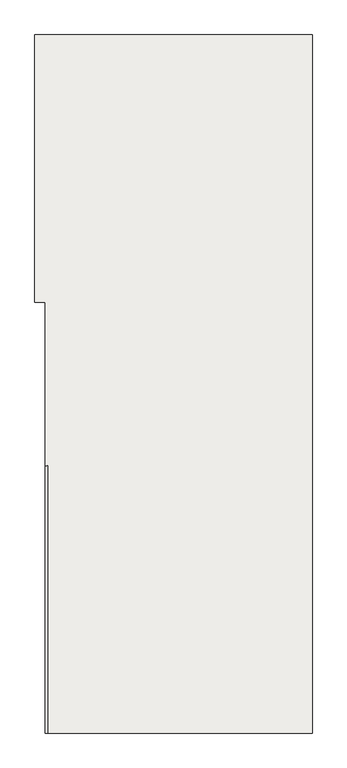
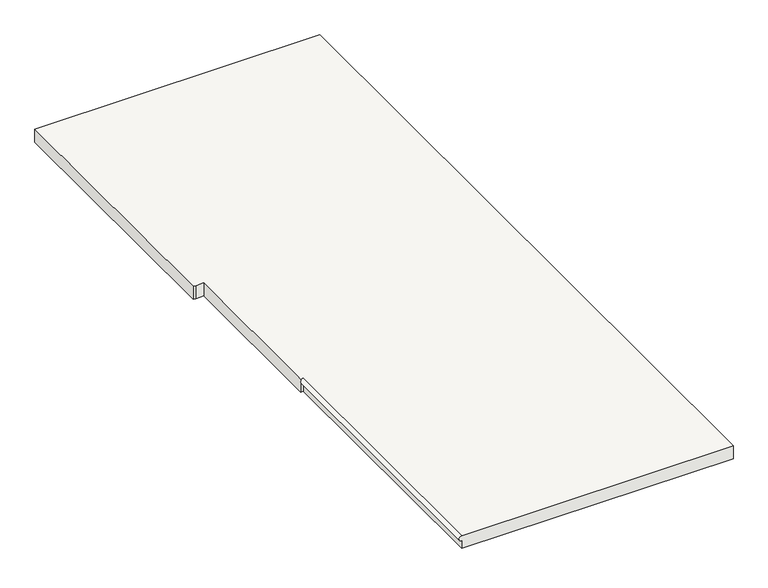
"""IFC4 building model written with IfcOpenShell, lengths in millimetres: slab geometry."""

from ifc_helpers import new_model, si_unit, frame, origin, place, context, project, spatial, circle_curve, source, transform, mapped, element, save
from ifc_brep_helpers import plane_surface, cylinder_surface, advanced_brep


def slab_9cf16a29(model_context):
    return source(origin(), model_context, "Body", "AdvancedBrep", [
        advanced_brep(
        [(2455.490348, 19.7308056, 2630.3647059), (2455.490348, 19.7308056, 2650.3647059), (2455.490348, 1019.7308056, 2650.3647059), (2445.490348, 1019.7308056, 2640.3647059), (2455.490348, 1019.7308056, 2630.3647059), (2445.490348, 1019.7308056, 2650.3647059), (3445.490348, 19.7308056, 2650.3647059), (3445.490348, 2631.1308056, 2650.3647059), (2416.940348, 2631.1308056, 2650.3647059), (2406.940348, 2631.1308056, 2650.3647059), (2406.940348, 1631.1308056, 2650.3647059), (2416.940348, 1631.1308056, 2650.3647059), (2445.490348, 1631.1308056, 2650.3647059), (2455.490348, 1019.7308056, 2600.3647059), (2445.490348, 1019.7308056, 2600.3647059), (2445.490348, 1631.1308056, 2600.3647059), (2416.940348, 1631.1308056, 2600.3647059), (2406.940348, 1631.1308056, 2600.3647059), (2406.940348, 2631.1308056, 2600.3647059), (2416.940348, 2631.1308056, 2600.3647059), (3445.490348, 2631.1308056, 2600.3647059), (3445.490348, 19.7308056, 2600.3647059), (2455.490348, 19.7308056, 2600.3647059)],
        [
            (0, 1, circle_curve(frame((2455.490348, 19.7308056, 2640.3647059), z_axis=(0.0, 1.0, 0.0), x_axis=(1.0, 0.0, 0.0)), 10.0)),
            (1, 2),
            (2, 3, circle_curve(frame((2455.490348, 1019.7308056, 2640.3647059), z_axis=(0.0, -1.0, 0.0), x_axis=(1.0, 0.0, 0.0)), 10.0)),
            (3, 4, circle_curve(frame((2455.490348, 1019.7308056, 2640.3647059), z_axis=(0.0, -1.0, 0.0), x_axis=(1.0, 0.0, 0.0)), 10.0)),
            (4, 0),
            (5, 2),
            (1, 6),
            (6, 7),
            (7, 8),
            (8, 9),
            (9, 10),
            (10, 11),
            (11, 12),
            (12, 5),
            (13, 14),
            (14, 15),
            (15, 16),
            (16, 17),
            (17, 18),
            (18, 19),
            (19, 20),
            (20, 21),
            (21, 22),
            (22, 13),
            (5, 3),
            (13, 4),
            (3, 14),
            (22, 0),
            (21, 6),
            (20, 7),
            (19, 8),
            (18, 9),
            (17, 10),
            (16, 11),
            (15, 12),
        ],
        [
            cylinder_surface(frame((2455.490348, 19.7308056, 2640.3647059), z_axis=(0.0, -1.0, 0.0), x_axis=(1.0, 0.0, 0.0)), 10.0),
            plane_surface(frame((2445.490348, 1019.7308056, 2650.3647059), z_axis=(0.0, 0.0, 1.0), x_axis=(1.0, 0.0, 0.0))),
            plane_surface(frame((2445.490348, 1019.7308056, 2600.3647059), z_axis=(0.0, 0.0, -1.0), x_axis=(-1.0, 0.0, 0.0))),
            plane_surface(frame((2445.490348, 1019.7308056, 2650.3647059), z_axis=(0.0, -1.0, 0.0), x_axis=(0.0, 0.0, -1.0))),
            plane_surface(frame((2455.490348, 1019.7308056, 2650.3647059), z_axis=(-1.0, 0.0, 0.0), x_axis=(0.0, 0.0, -1.0))),
            plane_surface(frame((2455.490348, 19.7308056, 2650.3647059), z_axis=(0.0, -1.0, 0.0), x_axis=(0.0, 0.0, -1.0))),
            plane_surface(frame((3445.490348, 19.7308056, 2650.3647059), z_axis=(1.0, 0.0, 0.0), x_axis=(0.0, 0.0, -1.0))),
            plane_surface(frame((3445.490348, 2631.1308056, 2650.3647059), z_axis=(0.0, 1.0, 0.0), x_axis=(0.0, 0.0, -1.0))),
            plane_surface(frame((2416.940348, 2631.1308056, 2650.3647059), z_axis=(0.0, 1.0, 0.0), x_axis=(0.0, 0.0, -1.0))),
            plane_surface(frame((2406.940348, 2631.1308056, 2650.3647059), z_axis=(-1.0, 0.0, 0.0), x_axis=(0.0, 0.0, -1.0))),
            plane_surface(frame((2406.940348, 1631.1308056, 2650.3647059), z_axis=(0.0, -1.0, 0.0), x_axis=(0.0, 0.0, -1.0))),
            plane_surface(frame((2416.940348, 1631.1308056, 2650.3647059), z_axis=(0.0, -1.0, 0.0), x_axis=(0.0, 0.0, -1.0))),
            plane_surface(frame((2445.490348, 1631.1308056, 2650.3647059), z_axis=(-1.0, 0.0, 0.0), x_axis=(0.0, 0.0, -1.0))),
        ],
        [
            (0, [[1, 2, 3, 4, 5]]),
            (1, [[6, -2, 7, 8, 9, 10, 11, 12, 13, 14]]),
            (2, [[15, 16, 17, 18, 19, 20, 21, 22, 23, 24]]),
            (3, [[-6, 25, -3]]),
            (3, [[-15, 26, -4, 27]]),
            (4, [[-24, 28, -5, -26]]),
            (5, [[-7, -1, -28, -23, 29]]),
            (6, [[-8, -29, -22, 30]]),
            (7, [[-9, -30, -21, 31]]),
            (8, [[-10, -31, -20, 32]]),
            (9, [[-11, -32, -19, 33]]),
            (10, [[-12, -33, -18, 34]]),
            (11, [[-13, -34, -17, 35]]),
            (12, [[-14, -35, -16, -27, -25]]),
        ],
    ),
    ])


if __name__ == "__main__":
    model = new_model("IFC4")
    model_context = context("Model", 3, world=origin())
    ifc_project = project(units=[si_unit("LENGTHUNIT", "METRE", prefix="MILLI")], contexts=[model_context])
    site = spatial("IfcSite", under=ifc_project)
    building = spatial("IfcBuilding", under=site)
    placement = place(None, origin())
    slab_shape = slab_9cf16a29(model_context)
    element("IfcSlab", 1, at=placement, inside=building, context=model_context, shape_type="MappedRepresentation", body=[
        mapped(slab_shape, transform((0.0, 0.0, 0.0), x_axis=(1.0, 0.0, 0.0), y_axis=(0.0, 1.0, 0.0), z_axis=(0.0, 0.0, 1.0))),
    ])
    save(model, "model.ifc")

# Revit data of these elements
# Element 1 (IfcSlab)
#   Materials on its faces: "Oak Flooring"
# Materials
#   "Oak Flooring": class "Wood", colour RGB 212 179 113, transparency 0, Description = "Quercus Rubra", Cost = 0
